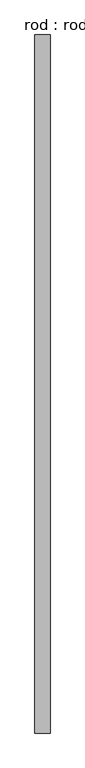
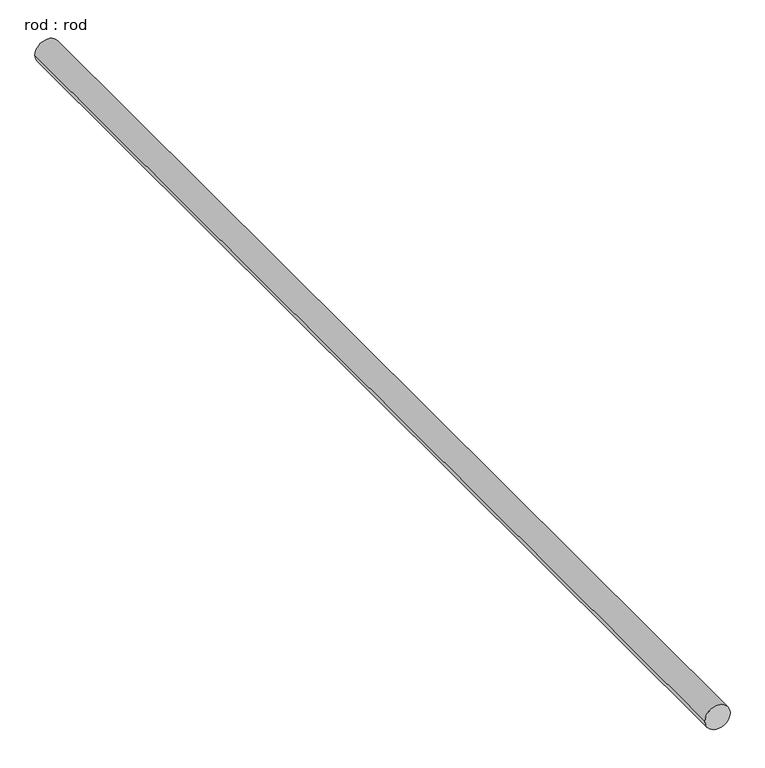
"""IFC4 building model written with IfcOpenShell, lengths in millimetres: proxy geometry, rod : rod."""

import ifcopenshell
import ifcopenshell.guid

model = None  # the IFC model being written
_history = None  # IfcOwnerHistory: only IFC2X3 demands one
_inside = {}  # id of a spatial element -> (the spatial element, [elements in it])
_under = {}  # id of a project, library or spatial element -> (it, [spatial elements below it])
_declared = {}  # id of a project -> (the project, [libraries it declares])
_typed = {}  # id of a type object -> (the type object, [elements of that type])
_made_of = {}  # id of a material, layer set ... -> (it, [elements and type objects made of it])


def new_model(schema):
    """Start an empty IFC model of exactly this schema.

    Asked for "IFC4X3", IfcOpenShell would pick the latest addendum, in which some entities
    have other attributes; the version numbers below select the first issue.
    IFC2X3 requires an IfcOwnerHistory on every rooted entity: one is made here for all.
    """
    global model, _history
    if schema == "IFC4X3":
        model = ifcopenshell.file(schema_version=(4, 3, 0, 0))
    else:
        model = ifcopenshell.file(schema=schema)
    _inside.clear()
    _under.clear()
    _declared.clear()
    _typed.clear()
    _made_of.clear()
    _history = None
    if model.schema == "IFC2X3":
        org = make("IfcOrganization", Name="unknown")
        user = make(
            "IfcPersonAndOrganization",
            ThePerson=make("IfcPerson", FamilyName="unknown"),
            TheOrganization=org,
        )
        app = make(
            "IfcApplication",
            ApplicationDeveloper=org,
            Version="unknown",
            ApplicationFullName="unknown",
            ApplicationIdentifier="unknown",
        )
        _history = make(
            "IfcOwnerHistory",
            OwningUser=user,
            OwningApplication=app,
            ChangeAction="ADDED",
            CreationDate=0,
        )
    return model


def make(cls, **values):
    """One entity of the class cls with the attributes given. An attribute that is None is left unset."""
    return model.create_entity(
        cls, **{name: value for name, value in values.items() if value is not None}
    )


def rooted(cls, **values):
    """An entity with a GlobalId (a new one), such as an element, a storey or a relation."""
    return make(cls, GlobalId=ifcopenshell.guid.new(), OwnerHistory=_history, **values)


def si_unit(unit_type, name, prefix=None):
    """IfcSIUnit, for example si_unit("LENGTHUNIT", "METRE", prefix="MILLI")."""
    return make("IfcSIUnit", UnitType=unit_type, Prefix=prefix, Name=name)


def assignment(units):
    """IfcUnitAssignment: the units of a project."""
    return None if units is None else make("IfcUnitAssignment", Units=units)


def point(xyz):
    """IfcCartesianPoint."""
    return None if xyz is None else make("IfcCartesianPoint", Coordinates=xyz)


def direction(xyz):
    """IfcDirection."""
    return None if xyz is None else make("IfcDirection", DirectionRatios=xyz)


def frame(location, z_axis=None, x_axis=None):
    """IfcAxis2Placement3D, a coordinate frame: its origin and axes. An axis left out is left unset."""
    return make(
        "IfcAxis2Placement3D",
        Location=point(location),
        Axis=direction(z_axis),
        RefDirection=direction(x_axis),
    )


def frame_2d(location, x_axis=None):
    """IfcAxis2Placement2D, a coordinate frame in the plane: its origin and x axis."""
    return make(
        "IfcAxis2Placement2D", Location=point(location), RefDirection=direction(x_axis)
    )


def origin():
    """The frame at (0, 0, 0) with its axes left unset."""
    return frame((0.0, 0.0, 0.0))


def place(relative_to, where):
    """IfcLocalPlacement: puts the frame where relative to a parent placement (None: the world)."""
    return make(
        "IfcLocalPlacement", PlacementRelTo=relative_to, RelativePlacement=where
    )


def context(
    kind, dimensions, precision=None, world=None, true_north=None, identifier=None
):
    """IfcGeometricRepresentationContext, for example the 3D "Model" context."""
    return make(
        "IfcGeometricRepresentationContext",
        ContextIdentifier=identifier,
        ContextType=kind,
        CoordinateSpaceDimension=dimensions,
        Precision=precision,
        WorldCoordinateSystem=world,
        TrueNorth=true_north,
    )


def project(units=None, contexts=None):
    """IfcProject with its units and contexts."""
    return rooted(
        "IfcProject",
        Name="project",
        RepresentationContexts=contexts,
        UnitsInContext=assignment(units),
    )


def spatial(cls, under=None, at=None, **own):
    """A site, building, storey or space (cls), placed at a placement, below another one or the project."""
    s = rooted(cls, ObjectPlacement=at, **own)
    if under is not None:
        _under.setdefault(under.id(), (under, []))[1].append(s)
    return s


def circle_curve(where, radius):
    """IfcCircle in the frame where."""
    return make("IfcCircle", Position=where, Radius=radius)


def trimmed(basis, trim1, trim2, sense, master):
    """IfcTrimmedCurve: the piece of a basis curve between two trims."""
    return make(
        "IfcTrimmedCurve",
        BasisCurve=basis,
        Trim1=trim1,
        Trim2=trim2,
        SenseAgreement=sense,
        MasterRepresentation=master,
    )


def segment(curve, same_sense, transition):
    """IfcCompositeCurveSegment."""
    return make(
        "IfcCompositeCurveSegment",
        Transition=transition,
        SameSense=same_sense,
        ParentCurve=curve,
    )


def composite_curve(segments, self_intersect=None):
    """IfcCompositeCurve: segments joined end to end."""
    return make("IfcCompositeCurve", Segments=segments, SelfIntersect=self_intersect)


def outline(outer, holes=None, kind="AREA"):
    """IfcArbitraryClosedProfileDef: a profile drawn as a closed curve; with holes, ...WithVoids."""
    if holes is None:
        return make("IfcArbitraryClosedProfileDef", ProfileType=kind, OuterCurve=outer)
    return make(
        "IfcArbitraryProfileDefWithVoids",
        ProfileType=kind,
        OuterCurve=outer,
        InnerCurves=holes,
    )


def extrude(swept, where, along, depth):
    """IfcExtrudedAreaSolid: the profile swept, set in the frame where, extruded along a direction by depth."""
    return make(
        "IfcExtrudedAreaSolid",
        SweptArea=swept,
        Position=where,
        ExtrudedDirection=direction(along),
        Depth=depth,
    )


def shape(context_of_items, identifier, shape_type, items):
    """IfcShapeRepresentation: the items that make up one representation, for example the "Body"."""
    return make(
        "IfcShapeRepresentation",
        ContextOfItems=context_of_items,
        RepresentationIdentifier=identifier,
        RepresentationType=shape_type,
        Items=items,
    )


def source(mapping_origin, context_of_items, identifier, shape_type, items):
    """IfcRepresentationMap: a shape defined once, which mapped items show again and again."""
    return make(
        "IfcRepresentationMap",
        MappingOrigin=mapping_origin,
        MappedRepresentation=shape(context_of_items, identifier, shape_type, items),
    )


def transform(
    local_origin,
    x_axis=None,
    y_axis=None,
    z_axis=None,
    scale=None,
    scale2=None,
    scale3=None,
    uniform=True,
):
    """IfcCartesianTransformationOperator3D, or its non-uniform kind. x_axis, y_axis, z_axis: its Axis1, 2, 3."""
    if uniform:
        return make(
            "IfcCartesianTransformationOperator3D",
            Axis1=direction(x_axis),
            Axis2=direction(y_axis),
            LocalOrigin=point(local_origin),
            Scale=scale,
            Axis3=direction(z_axis),
        )
    return make(
        "IfcCartesianTransformationOperator3DnonUniform",
        Axis1=direction(x_axis),
        Axis2=direction(y_axis),
        LocalOrigin=point(local_origin),
        Scale=scale,
        Axis3=direction(z_axis),
        Scale2=scale2,
        Scale3=scale3,
    )


def mapped(mapping_source, mapping_target):
    """IfcMappedItem: shows the shape of a source again, moved by a transform."""
    return make(
        "IfcMappedItem", MappingSource=mapping_source, MappingTarget=mapping_target
    )


def made_of(thing, what):
    """Note that an element or type object is made of a material, layer set ...; save() writes the relation."""
    if what is not None:
        _made_of.setdefault(what.id(), (what, []))[1].append(thing)
    return thing


def element(
    cls,
    number,
    at=None,
    inside=None,
    cuts=None,
    type_object=None,
    material=None,
    context=None,
    identifier="Body",
    shape_type=None,
    held_by="IfcProductDefinitionShape",
    body=None,
    shapes=None,
    **own,
):
    """One element of the class cls, such as IfcWall. Its Tag is "e" and its number.

    at: its placement. inside: the storey or other place that contains it. cuts: it is an
    opening in that element (IfcRelVoidsElement). A single representation is given by context,
    identifier, shape_type and body (its items); several are given by shapes. held_by: the class
    of the entity that holds the representations. save() writes the other relations.
    """
    e = rooted(cls, Tag="e%d" % number, ObjectPlacement=at, **own)
    if body is not None:
        shapes = [shape(context, identifier, shape_type, body)]
    if shapes is not None:
        e.Representation = make(held_by, Representations=shapes)
    if inside is not None:
        _inside.setdefault(inside.id(), (inside, []))[1].append(e)
    if cuts is not None:
        rooted(
            "IfcRelVoidsElement", RelatingBuildingElement=cuts, RelatedOpeningElement=e
        )
    if type_object is not None:
        _typed.setdefault(type_object.id(), (type_object, []))[1].append(e)
    return made_of(e, material)


def aggregate(whole, parts):
    """IfcRelAggregates: a whole, such as a stair, and the parts it consists of."""
    return rooted("IfcRelAggregates", RelatingObject=whole, RelatedObjects=parts)


def save(model, path):
    """Write the relations noted so far, then the file.

    IfcRelAggregates (storeys below a building ...), IfcRelContainedInSpatialStructure (elements
    in a storey), IfcRelDefinesByType, IfcRelAssociatesMaterial and IfcRelDeclares: one each for
    every whole, place, type object, material and project.
    """
    for whole, parts in _under.values():
        aggregate(whole, parts)
    for where, things in _inside.values():
        rooted(
            "IfcRelContainedInSpatialStructure",
            RelatedElements=things,
            RelatingStructure=where,
        )
    for kind, things in _typed.values():
        rooted("IfcRelDefinesByType", RelatedObjects=things, RelatingType=kind)
    for what, things in _made_of.values():
        rooted("IfcRelAssociatesMaterial", RelatedObjects=things, RelatingMaterial=what)
    for by, libraries in _declared.values():
        rooted("IfcRelDeclares", RelatingContext=by, RelatedDefinitions=libraries)
    model.write(path)


def rod_rod_5a06d1f6(model_context):
    return source(origin(), model_context, "Body", "SweptSolid", [
        extrude(outline(composite_curve([segment(trimmed(circle_curve(frame_2d((0.0108462, 0.0)), 200.0), [point((0.0108462, 200.0))], [point((0.0108462, -200.0))], False, "CARTESIAN"), True, "CONTINUOUS"), segment(trimmed(circle_curve(frame_2d((0.0108462, 0.0)), 200.0), [point((0.0108462, -200.0))], [point((0.0108462, 200.0))], False, "CARTESIAN"), True, "CONTINUOUS")], self_intersect=False)), frame((0.0, -5141.2199577, 0.0), z_axis=(0.0, 1.0, 0.0), x_axis=(0.0, 0.0, 1.0)), (0.0, 0.0, 1.0), 18467.8971461),
    ])


if __name__ == "__main__":
    model = new_model("IFC4")
    model_context = context("Model", 3, world=origin())
    ifc_project = project(units=[si_unit("LENGTHUNIT", "METRE", prefix="MILLI")], contexts=[model_context])
    site = spatial("IfcSite", under=ifc_project)
    building = spatial("IfcBuilding", under=site)
    placement = place(None, origin())
    rod_rod_shape = rod_rod_5a06d1f6(model_context)
    element("IfcBuildingElementProxy", 1, Name="rod : rod", ObjectType="rod : rod", at=placement, inside=building, context=model_context, shape_type="MappedRepresentation", body=[
        mapped(rod_rod_shape, transform((0.0, 0.0, 0.0), x_axis=(1.0, 0.0, 0.0), y_axis=(0.0, 1.0, 0.0), z_axis=(0.0, 0.0, 1.0))),
    ])
    save(model, "model.ifc")

# Revit data of these elements
# Type "rod : rod"
#   Default Elevation = 0
